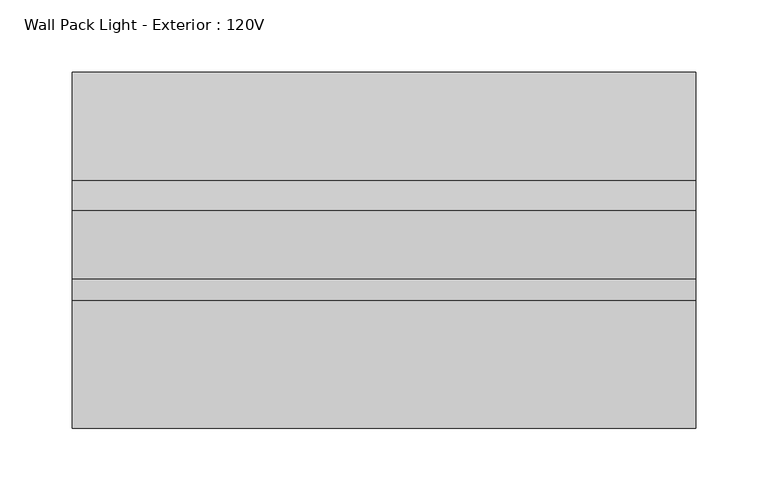
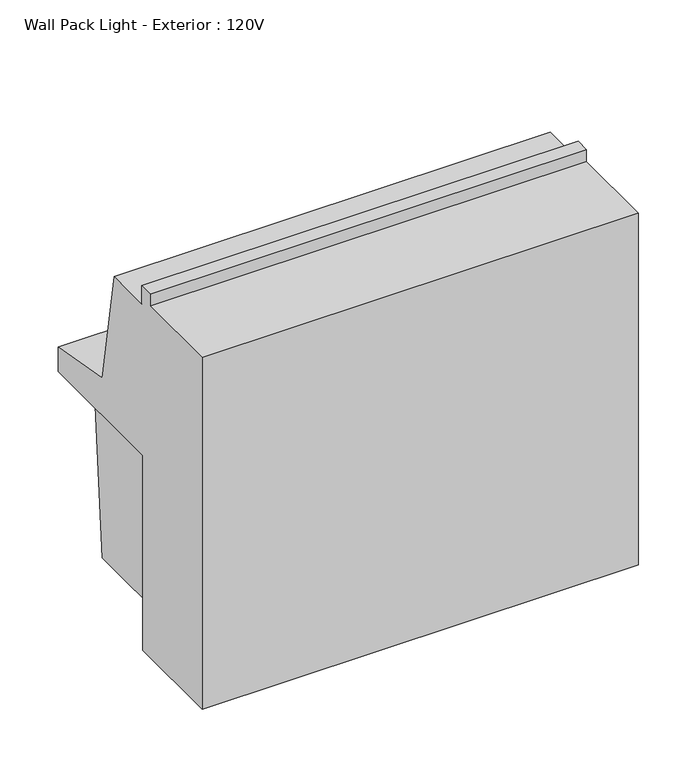
"""IFC4 building model written with IfcOpenShell, lengths in millimetres: light fixture geometry, Wall Pack Light - Exterior : 120V."""

from ifc_helpers import new_model, si_unit, frame, origin, place, context, project, spatial, polyline, outline, extrude, source, transform, mapped, element, save


def wall_pack_light_exterior_120v_dc6d378c(model_context):
    return source(origin(), model_context, "Body", "SweptSolid", [
        extrude(outline(polyline([(315.020745, 2393.95), (201.6, 2393.95), (201.6, 2578.1), (330.1170754, 2578.1), (315.020745, 2393.95)])), frame((-68.7349223, 0.0, 0.0), z_axis=(1.0, 0.0, 0.0), x_axis=(0.0, 1.0, 0.0)), (0.0, 0.0, 1.0), 380.9989788),
        extrude(outline(polyline([(188.9, 2755.9), (203.2, 2755.9), (203.2, 2736.85), (250.640971, 2736.85), (271.6426549, 2617.7435323), (346.6850056, 2604.5115412), (346.6850056, 2579.1115412), (201.6, 2579.1115412), (201.6, 2374.9), (100.0, 2374.9), (100.0, 2743.2), (188.9, 2743.2), (188.9, 2755.9)])), frame((-94.1359435, 0.0, 0.0), z_axis=(1.0, 0.0, 0.0), x_axis=(0.0, 1.0, 0.0)), (0.0, 0.0, 1.0), 431.8),
    ])


if __name__ == "__main__":
    model = new_model("IFC4")
    model_context = context("Model", 3, world=origin())
    ifc_project = project(units=[si_unit("LENGTHUNIT", "METRE", prefix="MILLI")], contexts=[model_context])
    site = spatial("IfcSite", under=ifc_project)
    building = spatial("IfcBuilding", under=site)
    placement = place(None, origin())
    wall_pack_light_exterior_120v_shape = wall_pack_light_exterior_120v_dc6d378c(model_context)
    element("IfcLightFixture", 1, ObjectType="Wall Pack Light - Exterior : 120V", at=placement, inside=building, context=model_context, shape_type="MappedRepresentation", body=[
        mapped(wall_pack_light_exterior_120v_shape, transform((0.0, 0.0, 0.0), x_axis=(1.0, 0.0, 0.0), y_axis=(0.0, 1.0, 0.0), z_axis=(0.0, 0.0, 1.0))),
    ])
    save(model, "model.ifc")

# Revit data of these elements
# Type "Wall Pack Light - Exterior : 120V"
#   Assembly Code = "D5020230"
#   Wattage = 70 W
#   built-in parameter 1150110 = 1 (stored number, unit not read)
#   built-in parameter 1114217 = 1 (stored number, unit not read)
#   built-in parameter 1150109 = 1 (stored number, unit not read)
#   built-in parameter 1150113 = 1 (stored number, unit not read)
#   built-in parameter 1150115 = 1 (stored number, unit not read)
#   built-in parameter 1150105 = 437.668 (stored number, unit not read)
#   Light Source Symbol Size = 0.6096 m
#   built-in parameter 1150112 = 1 (stored number, unit not read)
#   built-in parameter 1150114 = 1 (stored number, unit not read)
#   built-in parameter 1150107 = 4000 (stored number, unit not read)
#   built-in parameter 1150106 = 4.37668 (stored number, unit not read)
#   built-in parameter 1150104 = 7.29939 (stored number, unit not read)
#   Ballast Voltage = 120 V
#   built-in parameter 1114218 = 1 (stored number, unit not read)
#   built-in parameter 1150133 = 10 (stored number, unit not read)
#   Lumens = 5499.9 lm
#   Mounting Height = 2.7432 m
#   Apparent Load = 70 VA
#   built-in parameter 1150134 = 12
#   built-in parameter 1150137 = 1
#   Color Filter = 65535
#   Ballast Number of Poles = 1
#   Wall Mount Material = Metal - Paint Finish - Dark Grey, Matte
#   Shade Material = Glass
#   Load Classification = Lighting - Exterior
#   Dimming Lamp Color Temperature Shift = (empty or 0)
#   Default Elevation = 0
# Element 1 (IfcLightFixture, "Wall Pack Light - Exterior : 120V")
#   Materials on its faces: "Metal - Paint Finish - Dark Grey, Matte", "Glass"
# Materials
#   "Metal - Paint Finish - Dark Grey, Matte": class "Paint", colour RGB 98 98 98, transparency 0
#   "Glass": class "Glass", colour RGB 0 128 192, transparency 0.9, Description = "Soda Lime Glass", Cost = 0
